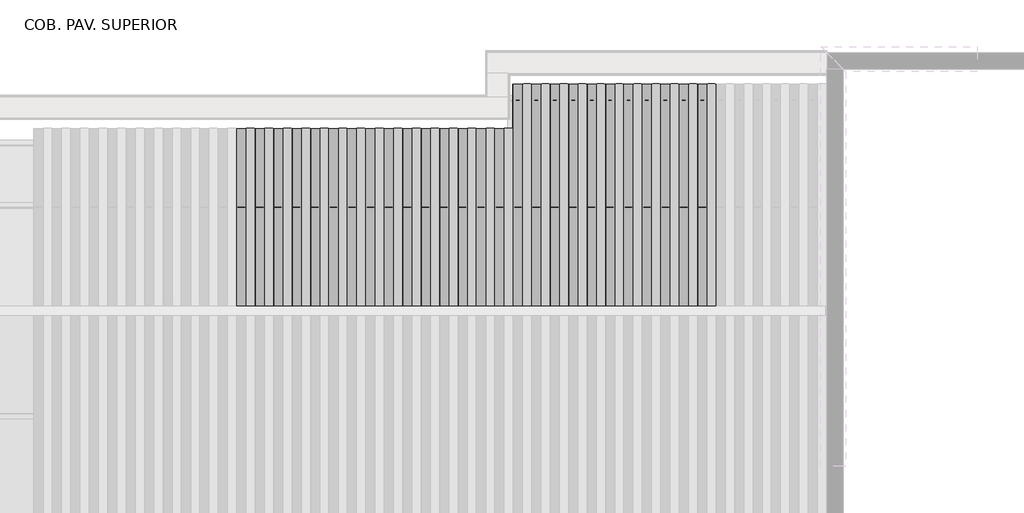
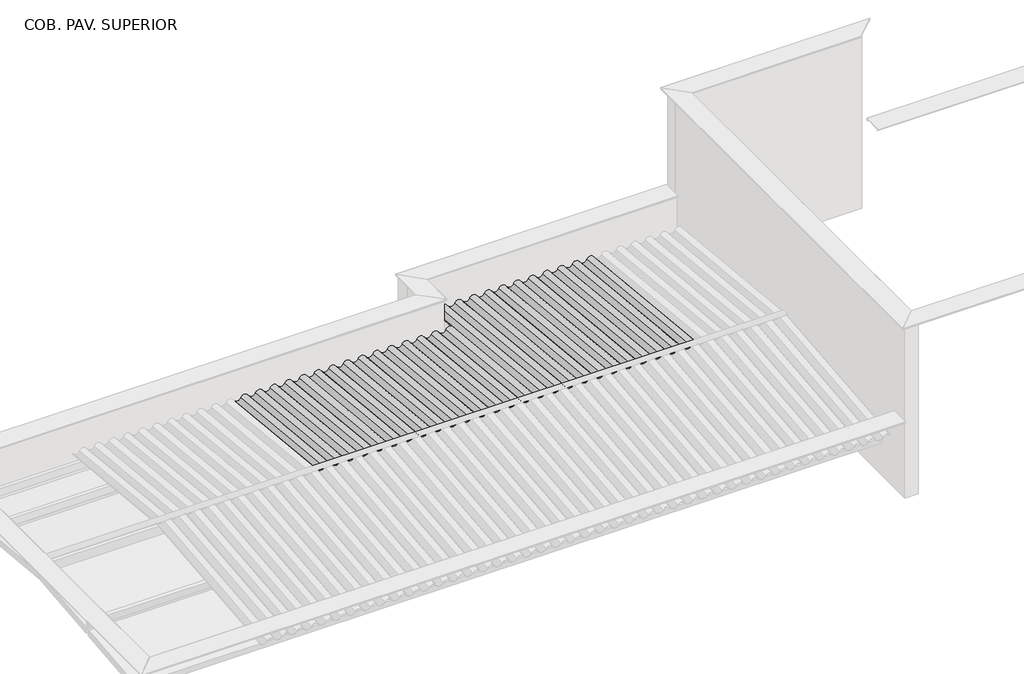
# One storey, part 4 of 7: 35 beams, 8 columns.
"""IFC4 building model written with IfcOpenShell, lengths in millimetres."""

import ifcopenshell
import ifcopenshell.guid

model = None  # the IFC model being written
_history = None  # IfcOwnerHistory: only IFC2X3 demands one
_inside = {}  # id of a spatial element -> (the spatial element, [elements in it])
_under = {}  # id of a project, library or spatial element -> (it, [spatial elements below it])
_declared = {}  # id of a project -> (the project, [libraries it declares])
_typed = {}  # id of a type object -> (the type object, [elements of that type])
_made_of = {}  # id of a material, layer set ... -> (it, [elements and type objects made of it])


def new_model(schema):
    """Start an empty IFC model of exactly this schema.

    Asked for "IFC4X3", IfcOpenShell would pick the latest addendum, in which some entities
    have other attributes; the version numbers below select the first issue.
    IFC2X3 requires an IfcOwnerHistory on every rooted entity: one is made here for all.
    """
    global model, _history
    if schema == "IFC4X3":
        model = ifcopenshell.file(schema_version=(4, 3, 0, 0))
    else:
        model = ifcopenshell.file(schema=schema)
    _inside.clear()
    _under.clear()
    _declared.clear()
    _typed.clear()
    _made_of.clear()
    _history = None
    if model.schema == "IFC2X3":
        org = make("IfcOrganization", Name="unknown")
        user = make(
            "IfcPersonAndOrganization",
            ThePerson=make("IfcPerson", FamilyName="unknown"),
            TheOrganization=org,
        )
        app = make(
            "IfcApplication",
            ApplicationDeveloper=org,
            Version="unknown",
            ApplicationFullName="unknown",
            ApplicationIdentifier="unknown",
        )
        _history = make(
            "IfcOwnerHistory",
            OwningUser=user,
            OwningApplication=app,
            ChangeAction="ADDED",
            CreationDate=0,
        )
    return model


def make(cls, **values):
    """One entity of the class cls with the attributes given. An attribute that is None is left unset."""
    return model.create_entity(
        cls, **{name: value for name, value in values.items() if value is not None}
    )


def rooted(cls, **values):
    """An entity with a GlobalId (a new one), such as an element, a storey or a relation."""
    return make(cls, GlobalId=ifcopenshell.guid.new(), OwnerHistory=_history, **values)


def si_unit(unit_type, name, prefix=None):
    """IfcSIUnit, for example si_unit("LENGTHUNIT", "METRE", prefix="MILLI")."""
    return make("IfcSIUnit", UnitType=unit_type, Prefix=prefix, Name=name)


def assignment(units):
    """IfcUnitAssignment: the units of a project."""
    return None if units is None else make("IfcUnitAssignment", Units=units)


def point(xyz):
    """IfcCartesianPoint."""
    return None if xyz is None else make("IfcCartesianPoint", Coordinates=xyz)


def direction(xyz):
    """IfcDirection."""
    return None if xyz is None else make("IfcDirection", DirectionRatios=xyz)


def frame(location, z_axis=None, x_axis=None):
    """IfcAxis2Placement3D, a coordinate frame: its origin and axes. An axis left out is left unset."""
    return make(
        "IfcAxis2Placement3D",
        Location=point(location),
        Axis=direction(z_axis),
        RefDirection=direction(x_axis),
    )


def frame_2d(location, x_axis=None):
    """IfcAxis2Placement2D, a coordinate frame in the plane: its origin and x axis."""
    return make(
        "IfcAxis2Placement2D", Location=point(location), RefDirection=direction(x_axis)
    )


def origin():
    """The frame at (0, 0, 0) with its axes left unset."""
    return frame((0.0, 0.0, 0.0))


def place(relative_to, where):
    """IfcLocalPlacement: puts the frame where relative to a parent placement (None: the world)."""
    return make(
        "IfcLocalPlacement", PlacementRelTo=relative_to, RelativePlacement=where
    )


def context(
    kind, dimensions, precision=None, world=None, true_north=None, identifier=None
):
    """IfcGeometricRepresentationContext, for example the 3D "Model" context."""
    return make(
        "IfcGeometricRepresentationContext",
        ContextIdentifier=identifier,
        ContextType=kind,
        CoordinateSpaceDimension=dimensions,
        Precision=precision,
        WorldCoordinateSystem=world,
        TrueNorth=true_north,
    )


def project(units=None, contexts=None):
    """IfcProject with its units and contexts."""
    return rooted(
        "IfcProject",
        Name="project",
        RepresentationContexts=contexts,
        UnitsInContext=assignment(units),
    )


def spatial(cls, under=None, at=None, **own):
    """A site, building, storey or space (cls), placed at a placement, below another one or the project."""
    s = rooted(cls, ObjectPlacement=at, **own)
    if under is not None:
        _under.setdefault(under.id(), (under, []))[1].append(s)
    return s


def polyline(points):
    """IfcPolyline through the points."""
    return make("IfcPolyline", Points=[point(p) for p in points])


def circle_curve(where, radius):
    """IfcCircle in the frame where."""
    return make("IfcCircle", Position=where, Radius=radius)


def trimmed(basis, trim1, trim2, sense, master):
    """IfcTrimmedCurve: the piece of a basis curve between two trims."""
    return make(
        "IfcTrimmedCurve",
        BasisCurve=basis,
        Trim1=trim1,
        Trim2=trim2,
        SenseAgreement=sense,
        MasterRepresentation=master,
    )


def segment(curve, same_sense, transition):
    """IfcCompositeCurveSegment."""
    return make(
        "IfcCompositeCurveSegment",
        Transition=transition,
        SameSense=same_sense,
        ParentCurve=curve,
    )


def composite_curve(segments, self_intersect=None):
    """IfcCompositeCurve: segments joined end to end."""
    return make("IfcCompositeCurve", Segments=segments, SelfIntersect=self_intersect)


def outline(outer, holes=None, kind="AREA"):
    """IfcArbitraryClosedProfileDef: a profile drawn as a closed curve; with holes, ...WithVoids."""
    if holes is None:
        return make("IfcArbitraryClosedProfileDef", ProfileType=kind, OuterCurve=outer)
    return make(
        "IfcArbitraryProfileDefWithVoids",
        ProfileType=kind,
        OuterCurve=outer,
        InnerCurves=holes,
    )


def extrude(swept, where, along, depth):
    """IfcExtrudedAreaSolid: the profile swept, set in the frame where, extruded along a direction by depth."""
    return make(
        "IfcExtrudedAreaSolid",
        SweptArea=swept,
        Position=where,
        ExtrudedDirection=direction(along),
        Depth=depth,
    )


def shape(context_of_items, identifier, shape_type, items):
    """IfcShapeRepresentation: the items that make up one representation, for example the "Body"."""
    return make(
        "IfcShapeRepresentation",
        ContextOfItems=context_of_items,
        RepresentationIdentifier=identifier,
        RepresentationType=shape_type,
        Items=items,
    )


def source(mapping_origin, context_of_items, identifier, shape_type, items):
    """IfcRepresentationMap: a shape defined once, which mapped items show again and again."""
    return make(
        "IfcRepresentationMap",
        MappingOrigin=mapping_origin,
        MappedRepresentation=shape(context_of_items, identifier, shape_type, items),
    )


def transform(
    local_origin,
    x_axis=None,
    y_axis=None,
    z_axis=None,
    scale=None,
    scale2=None,
    scale3=None,
    uniform=True,
):
    """IfcCartesianTransformationOperator3D, or its non-uniform kind. x_axis, y_axis, z_axis: its Axis1, 2, 3."""
    if uniform:
        return make(
            "IfcCartesianTransformationOperator3D",
            Axis1=direction(x_axis),
            Axis2=direction(y_axis),
            LocalOrigin=point(local_origin),
            Scale=scale,
            Axis3=direction(z_axis),
        )
    return make(
        "IfcCartesianTransformationOperator3DnonUniform",
        Axis1=direction(x_axis),
        Axis2=direction(y_axis),
        LocalOrigin=point(local_origin),
        Scale=scale,
        Axis3=direction(z_axis),
        Scale2=scale2,
        Scale3=scale3,
    )


def mapped(mapping_source, mapping_target):
    """IfcMappedItem: shows the shape of a source again, moved by a transform."""
    return make(
        "IfcMappedItem", MappingSource=mapping_source, MappingTarget=mapping_target
    )


def made_of(thing, what):
    """Note that an element or type object is made of a material, layer set ...; save() writes the relation."""
    if what is not None:
        _made_of.setdefault(what.id(), (what, []))[1].append(thing)
    return thing


def element(
    cls,
    number,
    at=None,
    inside=None,
    cuts=None,
    type_object=None,
    material=None,
    context=None,
    identifier="Body",
    shape_type=None,
    held_by="IfcProductDefinitionShape",
    body=None,
    shapes=None,
    **own,
):
    """One element of the class cls, such as IfcWall. Its Tag is "e" and its number.

    at: its placement. inside: the storey or other place that contains it. cuts: it is an
    opening in that element (IfcRelVoidsElement). A single representation is given by context,
    identifier, shape_type and body (its items); several are given by shapes. held_by: the class
    of the entity that holds the representations. save() writes the other relations.
    """
    e = rooted(cls, Tag="e%d" % number, ObjectPlacement=at, **own)
    if body is not None:
        shapes = [shape(context, identifier, shape_type, body)]
    if shapes is not None:
        e.Representation = make(held_by, Representations=shapes)
    if inside is not None:
        _inside.setdefault(inside.id(), (inside, []))[1].append(e)
    if cuts is not None:
        rooted(
            "IfcRelVoidsElement", RelatingBuildingElement=cuts, RelatedOpeningElement=e
        )
    if type_object is not None:
        _typed.setdefault(type_object.id(), (type_object, []))[1].append(e)
    return made_of(e, material)


def aggregate(whole, parts):
    """IfcRelAggregates: a whole, such as a stair, and the parts it consists of."""
    return rooted("IfcRelAggregates", RelatingObject=whole, RelatedObjects=parts)


def save(model, path):
    """Write the relations noted so far, then the file.

    IfcRelAggregates (storeys below a building ...), IfcRelContainedInSpatialStructure (elements
    in a storey), IfcRelDefinesByType, IfcRelAssociatesMaterial and IfcRelDeclares: one each for
    every whole, place, type object, material and project.
    """
    for whole, parts in _under.values():
        aggregate(whole, parts)
    for where, things in _inside.values():
        rooted(
            "IfcRelContainedInSpatialStructure",
            RelatedElements=things,
            RelatingStructure=where,
        )
    for kind, things in _typed.values():
        rooted("IfcRelDefinesByType", RelatedObjects=things, RelatingType=kind)
    for what, things in _made_of.values():
        rooted("IfcRelAssociatesMaterial", RelatedObjects=things, RelatingMaterial=what)
    for by, libraries in _declared.values():
        rooted("IfcRelDeclares", RelatingContext=by, RelatedDefinitions=libraries)
    model.write(path)


def column_d505325c(model_context):
    return source(origin(), model_context, "Body", "SweptSolid", [
        extrude(outline(polyline([(30.0, 80.0), (30.0, -80.0), (-30.0, -80.0), (-30.0, 80.0), (30.0, 80.0)])), frame((0.0, 0.0, 6710.0), z_axis=(0.0, 0.0, 1.0), x_axis=(1.0, 0.0, 0.0)), (0.0, 0.0, 1.0), 750.0),
    ])


def column_df674f92(model_context):
    return source(origin(), model_context, "Body", "SweptSolid", [
        extrude(outline(polyline([(30.0, 80.0), (30.0, -80.0), (-30.0, -80.0), (-30.0, 80.0), (30.0, 80.0)])), frame((0.0, 0.0, 6710.0), z_axis=(0.0, 0.0, 1.0), x_axis=(1.0, 0.0, 0.0)), (0.0, 0.0, 1.0), 575.0),
    ])


def column_4db371bd(model_context):
    return source(origin(), model_context, "Body", "SweptSolid", [
        extrude(outline(polyline([(30.0, 80.0), (30.0, -80.0), (-30.0, -80.0), (-30.0, 80.0), (30.0, 80.0)])), frame((0.0, 0.0, 6710.0), z_axis=(0.0, 0.0, 1.0), x_axis=(1.0, 0.0, 0.0)), (0.0, 0.0, 1.0), 660.0),
    ])


model = new_model("IFC4")

# Units and contexts
model_context = context("Model", 3, world=origin())
ifc_project = project(units=[si_unit("LENGTHUNIT", "METRE", prefix="MILLI")], contexts=[model_context])

# Site, building, storey
site = spatial("IfcSite", under=ifc_project)
building = spatial("IfcBuilding", under=site)
storey = spatial("IfcBuildingStorey", under=building, Name="COB. PAV. SUPERIOR", Elevation=6650.0)

# Beams
placement = place(None, origin())
element("IfcBeam", 1, ObjectType="Madeira de lei : Berço 6x12cm", at=placement, inside=storey, context=model_context, shape_type="SweptSolid", body=[
    extrude(outline(polyline([(-4679.281307, -7711.5607799), (-4679.281307, -7831.5607799), (-6679.281307, -7831.5607799), (-6679.281307, -7711.5607799), (-4679.281307, -7711.5607799)])), frame((0.0, 0.0, 6650.0), z_axis=(0.0, 0.0, 1.0), x_axis=(1.0, 0.0, 0.0)), (0.0, 0.0, 1.0), 60.0),
])
element("IfcBeam", 2, ObjectType="Madeira de lei : Berço 6x12cm", at=placement, inside=storey, context=model_context, shape_type="SweptSolid", body=[
    extrude(outline(polyline([(-2679.281307, -7711.5607799), (-2679.281307, -7831.5607799), (-4679.281307, -7831.5607799), (-4679.281307, -7711.5607799), (-2679.281307, -7711.5607799)])), frame((0.0, 0.0, 6650.0), z_axis=(0.0, 0.0, 1.0), x_axis=(1.0, 0.0, 0.0)), (0.0, 0.0, 1.0), 60.0),
])
element("IfcBeam", 3, ObjectType="Madeira de lei : Berço 6x12cm", at=placement, inside=storey, context=model_context, shape_type="SweptSolid", body=[
    extrude(outline(polyline([(-679.281307, -7711.5607799), (-679.281307, -7831.5607799), (-2679.281307, -7831.5607799), (-2679.281307, -7711.5607799), (-679.281307, -7711.5607799)])), frame((0.0, 0.0, 6650.0), z_axis=(0.0, 0.0, 1.0), x_axis=(1.0, 0.0, 0.0)), (0.0, 0.0, 1.0), 60.0),
])
element("IfcBeam", 4, ObjectType="Madeira de lei : Berço 6x12cm", at=placement, inside=storey, context=model_context, shape_type="SweptSolid", body=[
    extrude(outline(polyline([(-244.281307, -7711.5607799), (-244.281307, -7831.5607799), (-679.281307, -7831.5607799), (-679.281307, -7711.5607799), (-244.281307, -7711.5607799)])), frame((0.0, 0.0, 6650.0), z_axis=(0.0, 0.0, 1.0), x_axis=(1.0, 0.0, 0.0)), (0.0, 0.0, 1.0), 60.0),
])
element("IfcBeam", 5, ObjectType="Madeira de lei : Berço 6x12cm", at=placement, inside=storey, context=model_context, shape_type="SweptSolid", body=[
    extrude(outline(polyline([(-6779.2813076, -5488.3211004), (-6779.2813076, -5608.3211004), (-8589.281307, -5608.3211004), (-8589.281307, -5488.3211004), (-6779.2813076, -5488.3211004)])), frame((0.0, 0.0, 6650.0), z_axis=(0.0, 0.0, 1.0), x_axis=(1.0, 0.0, 0.0)), (0.0, 0.0, 1.0), 60.0),
])
element("IfcBeam", 6, ObjectType="Madeira de lei : Berço 6x12cm", at=placement, inside=storey, context=model_context, shape_type="SweptSolid", body=[
    extrude(outline(polyline([(-4779.281307, -5488.3211004), (-4779.281307, -5608.3211004), (-6779.2813063, -5608.3211004), (-6779.2813063, -5488.3211004), (-4779.281307, -5488.3211004)])), frame((0.0, 0.0, 6650.0), z_axis=(0.0, 0.0, 1.0), x_axis=(1.0, 0.0, 0.0)), (0.0, 0.0, 1.0), 60.0),
])
element("IfcBeam", 7, ObjectType="Madeira de lei : Berço 6x12cm", at=placement, inside=storey, context=model_context, shape_type="SweptSolid", body=[
    extrude(outline(polyline([(-6840.281307, -6319.8711004), (-6840.281307, -6439.8711004), (-8589.281307, -6439.8711004), (-8589.281307, -6319.8711004), (-6840.281307, -6319.8711004)])), frame((0.0, 0.0, 6650.0), z_axis=(0.0, 0.0, 1.0), x_axis=(1.0, 0.0, 0.0)), (0.0, 0.0, 1.0), 60.0),
])
element("IfcBeam", 8, ObjectType="Madeira de lei : Berço 6x12cm", at=placement, inside=storey, context=model_context, shape_type="SweptSolid", body=[
    extrude(outline(polyline([(-4679.2813076, -6319.8711004), (-4679.2813076, -6439.8711004), (-6440.281307, -6439.8711004), (-6440.281307, -6319.8711004), (-4679.2813076, -6319.8711004)])), frame((0.0, 0.0, 6650.0), z_axis=(0.0, 0.0, 1.0), x_axis=(1.0, 0.0, 0.0)), (0.0, 0.0, 1.0), 60.0),
])
element("IfcBeam", 9, ObjectType="Madeira de lei : Berço 6x12cm", at=placement, inside=storey, context=model_context, shape_type="SweptSolid", body=[
    extrude(outline(polyline([(-2679.2813076, -6319.8711004), (-2679.2813076, -6439.8711004), (-4679.2813064, -6439.8711004), (-4679.2813064, -6319.8711004), (-2679.2813076, -6319.8711004)])), frame((0.0, 0.0, 6650.0), z_axis=(0.0, 0.0, 1.0), x_axis=(1.0, 0.0, 0.0)), (0.0, 0.0, 1.0), 60.0),
])
element("IfcBeam", 10, ObjectType="Telha Ondulada : Fibrocimento", at=placement, inside=storey, context=model_context, shape_type="SweptSolid", body=[
    extrude(outline(composite_curve([segment(trimmed(circle_curve(frame_2d((-58.7002978, -53.2060539)), 66.7939461), [point((-29.3501489, 6.7939461))], [point((-29.3501489, -113.2060539))], False, "CARTESIAN"), True, "CONTINUOUS"), segment(polyline([(-29.3501489, -113.2060539), (-31.5472154, -108.7146289)]), True, "CONTINUOUS"), segment(trimmed(circle_curve(frame_2d((-58.7002978, -53.2060539)), 61.7939461), [point((-31.5472154, -108.7146289))], [point((-31.5472154, 2.3025211))], True, "CARTESIAN"), True, "CONTINUOUS"), segment(trimmed(circle_curve(frame_2d((0.0, 66.7939461)), 71.7939461), [point((-31.5472154, 2.3025211))], [point((-31.5472154, 131.2853711))], False, "CARTESIAN"), True, "CONTINUOUS"), segment(polyline([(-31.5472154, 131.2853711), (-29.3501489, 126.7939461)]), True, "CONTINUOUS"), segment(trimmed(circle_curve(frame_2d((0.0, 66.7939461)), 66.7939461), [point((-29.3501489, 126.7939461))], [point((-29.3501489, 6.7939461))], True, "CARTESIAN"), True, "CONTINUOUS")], self_intersect=False)), frame((-7939.8843743, -5348.1805671, 7453.4315886), z_axis=(0.0, -0.9950371902099893, 0.09950371902099772), x_axis=(0.0, 0.09950371902099772, 0.9950371902099893)), (0.0, 0.0, 1.0), 2425.2918406),
])
element("IfcBeam", 11, ObjectType="Telha Ondulada : Fibrocimento", at=placement, inside=storey, context=model_context, shape_type="SweptSolid", body=[
    extrude(outline(composite_curve([segment(trimmed(circle_curve(frame_2d((-58.7002978, -53.2060539)), 66.7939461), [point((-29.3501489, 6.7939461))], [point((-29.3501489, -113.2060539))], False, "CARTESIAN"), True, "CONTINUOUS"), segment(polyline([(-29.3501489, -113.2060539), (-31.5472154, -108.7146289)]), True, "CONTINUOUS"), segment(trimmed(circle_curve(frame_2d((-58.7002978, -53.2060539)), 61.7939461), [point((-31.5472154, -108.7146289))], [point((-31.5472154, 2.3025211))], True, "CARTESIAN"), True, "CONTINUOUS"), segment(trimmed(circle_curve(frame_2d((0.0, 66.7939461)), 71.7939461), [point((-31.5472154, 2.3025211))], [point((-31.5472154, 131.2853711))], False, "CARTESIAN"), True, "CONTINUOUS"), segment(polyline([(-31.5472154, 131.2853711), (-29.3501489, 126.7939461)]), True, "CONTINUOUS"), segment(trimmed(circle_curve(frame_2d((0.0, 66.7939461)), 66.7939461), [point((-29.3501489, 126.7939461))], [point((-29.3501489, 6.7939461))], True, "CARTESIAN"), True, "CONTINUOUS")], self_intersect=False)), frame((-7695.3843743, -5348.1805671, 7453.4315886), z_axis=(0.0, -0.9950371902099893, 0.09950371902099772), x_axis=(0.0, 0.09950371902099772, 0.9950371902099893)), (0.0, 0.0, 1.0), 2425.2918406),
])
element("IfcBeam", 12, ObjectType="Telha Ondulada : Fibrocimento", at=placement, inside=storey, context=model_context, shape_type="SweptSolid", body=[
    extrude(outline(composite_curve([segment(trimmed(circle_curve(frame_2d((-58.7002978, -53.2060539)), 66.7939461), [point((-29.3501489, 6.7939461))], [point((-29.3501489, -113.2060539))], False, "CARTESIAN"), True, "CONTINUOUS"), segment(polyline([(-29.3501489, -113.2060539), (-31.5472154, -108.7146289)]), True, "CONTINUOUS"), segment(trimmed(circle_curve(frame_2d((-58.7002978, -53.2060539)), 61.7939461), [point((-31.5472154, -108.7146289))], [point((-31.5472154, 2.3025211))], True, "CARTESIAN"), True, "CONTINUOUS"), segment(trimmed(circle_curve(frame_2d((0.0, 66.7939461)), 71.7939461), [point((-31.5472154, 2.3025211))], [point((-31.5472154, 131.2853711))], False, "CARTESIAN"), True, "CONTINUOUS"), segment(polyline([(-31.5472154, 131.2853711), (-29.3501489, 126.7939461)]), True, "CONTINUOUS"), segment(trimmed(circle_curve(frame_2d((0.0, 66.7939461)), 66.7939461), [point((-29.3501489, 126.7939461))], [point((-29.3501489, 6.7939461))], True, "CARTESIAN"), True, "CONTINUOUS")], self_intersect=False)), frame((-7450.8843743, -5348.1805671, 7453.4315886), z_axis=(0.0, -0.9950371902099893, 0.09950371902099768), x_axis=(0.0, 0.09950371902099768, 0.9950371902099893)), (0.0, 0.0, 1.0), 2425.2918406),
])
element("IfcBeam", 13, ObjectType="Telha Ondulada : Fibrocimento", at=placement, inside=storey, context=model_context, shape_type="SweptSolid", body=[
    extrude(outline(composite_curve([segment(trimmed(circle_curve(frame_2d((-58.7002978, -53.2060539)), 66.7939461), [point((-29.3501489, 6.7939461))], [point((-29.3501489, -113.2060539))], False, "CARTESIAN"), True, "CONTINUOUS"), segment(polyline([(-29.3501489, -113.2060539), (-31.5472154, -108.7146289)]), True, "CONTINUOUS"), segment(trimmed(circle_curve(frame_2d((-58.7002978, -53.2060539)), 61.7939461), [point((-31.5472154, -108.7146289))], [point((-31.5472154, 2.3025211))], True, "CARTESIAN"), True, "CONTINUOUS"), segment(trimmed(circle_curve(frame_2d((0.0, 66.7939461)), 71.7939461), [point((-31.5472154, 2.3025211))], [point((-31.5472154, 131.2853711))], False, "CARTESIAN"), True, "CONTINUOUS"), segment(polyline([(-31.5472154, 131.2853711), (-29.3501489, 126.7939461)]), True, "CONTINUOUS"), segment(trimmed(circle_curve(frame_2d((0.0, 66.7939461)), 66.7939461), [point((-29.3501489, 126.7939461))], [point((-29.3501489, 6.7939461))], True, "CARTESIAN"), True, "CONTINUOUS")], self_intersect=False)), frame((-7206.3843743, -5348.1805671, 7453.4315886), z_axis=(0.0, -0.9950371902099893, 0.09950371902099768), x_axis=(0.0, 0.09950371902099768, 0.9950371902099893)), (0.0, 0.0, 1.0), 2425.2918406),
])
element("IfcBeam", 14, ObjectType="Telha Ondulada : Fibrocimento", at=placement, inside=storey, context=model_context, shape_type="SweptSolid", body=[
    extrude(outline(composite_curve([segment(trimmed(circle_curve(frame_2d((-58.7002978, -53.2060539)), 66.7939461), [point((-29.3501489, 6.7939461))], [point((-29.3501489, -113.2060539))], False, "CARTESIAN"), True, "CONTINUOUS"), segment(polyline([(-29.3501489, -113.2060539), (-31.5472154, -108.7146289)]), True, "CONTINUOUS"), segment(trimmed(circle_curve(frame_2d((-58.7002978, -53.2060539)), 61.7939461), [point((-31.5472154, -108.7146289))], [point((-31.5472154, 2.3025211))], True, "CARTESIAN"), True, "CONTINUOUS"), segment(trimmed(circle_curve(frame_2d((0.0, 66.7939461)), 71.7939461), [point((-31.5472154, 2.3025211))], [point((-31.5472154, 131.2853711))], False, "CARTESIAN"), True, "CONTINUOUS"), segment(polyline([(-31.5472154, 131.2853711), (-29.3501489, 126.7939461)]), True, "CONTINUOUS"), segment(trimmed(circle_curve(frame_2d((0.0, 66.7939461)), 66.7939461), [point((-29.3501489, 126.7939461))], [point((-29.3501489, 6.7939461))], True, "CARTESIAN"), True, "CONTINUOUS")], self_intersect=False)), frame((-6961.8843743, -5348.1805671, 7453.4315886), z_axis=(0.0, -0.9950371902099893, 0.09950371902099768), x_axis=(0.0, 0.09950371902099768, 0.9950371902099893)), (0.0, 0.0, 1.0), 2425.2918406),
])
element("IfcBeam", 15, ObjectType="Telha Ondulada : Fibrocimento", at=placement, inside=storey, context=model_context, shape_type="SweptSolid", body=[
    extrude(outline(composite_curve([segment(trimmed(circle_curve(frame_2d((-58.7002978, -53.2060539)), 66.7939461), [point((-29.3501489, 6.7939461))], [point((-29.3501489, -113.2060539))], False, "CARTESIAN"), True, "CONTINUOUS"), segment(polyline([(-29.3501489, -113.2060539), (-31.5472154, -108.7146289)]), True, "CONTINUOUS"), segment(trimmed(circle_curve(frame_2d((-58.7002978, -53.2060539)), 61.7939461), [point((-31.5472154, -108.7146289))], [point((-31.5472154, 2.3025211))], True, "CARTESIAN"), True, "CONTINUOUS"), segment(trimmed(circle_curve(frame_2d((0.0, 66.7939461)), 71.7939461), [point((-31.5472154, 2.3025211))], [point((-31.5472154, 131.2853711))], False, "CARTESIAN"), True, "CONTINUOUS"), segment(polyline([(-31.5472154, 131.2853711), (-29.3501489, 126.7939461)]), True, "CONTINUOUS"), segment(trimmed(circle_curve(frame_2d((0.0, 66.7939461)), 66.7939461), [point((-29.3501489, 126.7939461))], [point((-29.3501489, 6.7939461))], True, "CARTESIAN"), True, "CONTINUOUS")], self_intersect=False)), frame((-6717.3843743, -5348.1805671, 7453.4315886), z_axis=(0.0, -0.9950371902099893, 0.09950371902099768), x_axis=(0.0, 0.09950371902099768, 0.9950371902099893)), (0.0, 0.0, 1.0), 2425.2918406),
])
element("IfcBeam", 16, ObjectType="Telha Ondulada : Fibrocimento", at=placement, inside=storey, context=model_context, shape_type="SweptSolid", body=[
    extrude(outline(composite_curve([segment(trimmed(circle_curve(frame_2d((-58.7002978, -53.2060539)), 66.7939461), [point((-29.3501489, 6.7939461))], [point((-29.3501489, -113.2060539))], False, "CARTESIAN"), True, "CONTINUOUS"), segment(polyline([(-29.3501489, -113.2060539), (-31.5472154, -108.7146289)]), True, "CONTINUOUS"), segment(trimmed(circle_curve(frame_2d((-58.7002978, -53.2060539)), 61.7939461), [point((-31.5472154, -108.7146289))], [point((-31.5472154, 2.3025211))], True, "CARTESIAN"), True, "CONTINUOUS"), segment(trimmed(circle_curve(frame_2d((0.0, 66.7939461)), 71.7939461), [point((-31.5472154, 2.3025211))], [point((-31.5472154, 131.2853711))], False, "CARTESIAN"), True, "CONTINUOUS"), segment(polyline([(-31.5472154, 131.2853711), (-29.3501489, 126.7939461)]), True, "CONTINUOUS"), segment(trimmed(circle_curve(frame_2d((0.0, 66.7939461)), 66.7939461), [point((-29.3501489, 126.7939461))], [point((-29.3501489, 6.7939461))], True, "CARTESIAN"), True, "CONTINUOUS")], self_intersect=False)), frame((-6472.8843743, -5348.1805671, 7453.4315886), z_axis=(0.0, -0.9950371902099893, 0.09950371902099772), x_axis=(0.0, 0.09950371902099772, 0.9950371902099893)), (0.0, 0.0, 1.0), 2425.2918406),
])
element("IfcBeam", 17, ObjectType="Telha Ondulada : Fibrocimento", at=placement, inside=storey, context=model_context, shape_type="SweptSolid", body=[
    extrude(outline(composite_curve([segment(trimmed(circle_curve(frame_2d((-58.7002978, -53.2060539)), 66.7939461), [point((-29.3501489, 6.7939461))], [point((-29.3501489, -113.2060539))], False, "CARTESIAN"), True, "CONTINUOUS"), segment(polyline([(-29.3501489, -113.2060539), (-31.5472154, -108.7146289)]), True, "CONTINUOUS"), segment(trimmed(circle_curve(frame_2d((-58.7002978, -53.2060539)), 61.7939461), [point((-31.5472154, -108.7146289))], [point((-31.5472154, 2.3025211))], True, "CARTESIAN"), True, "CONTINUOUS"), segment(trimmed(circle_curve(frame_2d((0.0, 66.7939461)), 71.7939461), [point((-31.5472154, 2.3025211))], [point((-31.5472154, 131.2853711))], False, "CARTESIAN"), True, "CONTINUOUS"), segment(polyline([(-31.5472154, 131.2853711), (-29.3501489, 126.7939461)]), True, "CONTINUOUS"), segment(trimmed(circle_curve(frame_2d((0.0, 66.7939461)), 66.7939461), [point((-29.3501489, 126.7939461))], [point((-29.3501489, 6.7939461))], True, "CARTESIAN"), True, "CONTINUOUS")], self_intersect=False)), frame((-6228.3843743, -5348.1805671, 7453.4315886), z_axis=(0.0, -0.9950371902099893, 0.09950371902099768), x_axis=(0.0, 0.09950371902099768, 0.9950371902099893)), (0.0, 0.0, 1.0), 2425.2918406),
])
element("IfcBeam", 18, ObjectType="Telha Ondulada : Fibrocimento", at=placement, inside=storey, context=model_context, shape_type="SweptSolid", body=[
    extrude(outline(composite_curve([segment(trimmed(circle_curve(frame_2d((-58.7002978, -53.2060539)), 66.7939461), [point((-29.3501489, 6.7939461))], [point((-29.3501489, -113.2060539))], False, "CARTESIAN"), True, "CONTINUOUS"), segment(polyline([(-29.3501489, -113.2060539), (-31.5472154, -108.7146289)]), True, "CONTINUOUS"), segment(trimmed(circle_curve(frame_2d((-58.7002978, -53.2060539)), 61.7939461), [point((-31.5472154, -108.7146289))], [point((-31.5472154, 2.3025211))], True, "CARTESIAN"), True, "CONTINUOUS"), segment(trimmed(circle_curve(frame_2d((0.0, 66.7939461)), 71.7939461), [point((-31.5472154, 2.3025211))], [point((-31.5472154, 131.2853711))], False, "CARTESIAN"), True, "CONTINUOUS"), segment(polyline([(-31.5472154, 131.2853711), (-29.3501489, 126.7939461)]), True, "CONTINUOUS"), segment(trimmed(circle_curve(frame_2d((0.0, 66.7939461)), 66.7939461), [point((-29.3501489, 126.7939461))], [point((-29.3501489, 6.7939461))], True, "CARTESIAN"), True, "CONTINUOUS")], self_intersect=False)), frame((-5983.8843743, -5348.1805671, 7453.4315886), z_axis=(0.0, -0.9950371902099893, 0.09950371902099772), x_axis=(0.0, 0.09950371902099772, 0.9950371902099893)), (0.0, 0.0, 1.0), 2425.2918406),
])
element("IfcBeam", 19, ObjectType="Telha Ondulada : Fibrocimento", at=placement, inside=storey, context=model_context, shape_type="SweptSolid", body=[
    extrude(outline(composite_curve([segment(trimmed(circle_curve(frame_2d((-58.7002978, -53.2060539)), 66.7939461), [point((-29.3501489, 6.7939461))], [point((-29.3501489, -113.2060539))], False, "CARTESIAN"), True, "CONTINUOUS"), segment(polyline([(-29.3501489, -113.2060539), (-31.5472154, -108.7146289)]), True, "CONTINUOUS"), segment(trimmed(circle_curve(frame_2d((-58.7002978, -53.2060539)), 61.7939461), [point((-31.5472154, -108.7146289))], [point((-31.5472154, 2.3025211))], True, "CARTESIAN"), True, "CONTINUOUS"), segment(trimmed(circle_curve(frame_2d((0.0, 66.7939461)), 71.7939461), [point((-31.5472154, 2.3025211))], [point((-31.5472154, 131.2853711))], False, "CARTESIAN"), True, "CONTINUOUS"), segment(polyline([(-31.5472154, 131.2853711), (-29.3501489, 126.7939461)]), True, "CONTINUOUS"), segment(trimmed(circle_curve(frame_2d((0.0, 66.7939461)), 66.7939461), [point((-29.3501489, 126.7939461))], [point((-29.3501489, 6.7939461))], True, "CARTESIAN"), True, "CONTINUOUS")], self_intersect=False)), frame((-5739.3843743, -5348.1805671, 7453.4315886), z_axis=(0.0, -0.9950371902099893, 0.09950371902099772), x_axis=(0.0, 0.09950371902099772, 0.9950371902099893)), (0.0, 0.0, 1.0), 2425.2918406),
])
element("IfcBeam", 20, ObjectType="Telha Ondulada : Fibrocimento", at=placement, inside=storey, context=model_context, shape_type="SweptSolid", body=[
    extrude(outline(composite_curve([segment(trimmed(circle_curve(frame_2d((-58.7002978, -53.2060539)), 66.7939461), [point((-29.3501489, 6.7939461))], [point((-29.3501489, -113.2060539))], False, "CARTESIAN"), True, "CONTINUOUS"), segment(polyline([(-29.3501489, -113.2060539), (-31.5472154, -108.7146289)]), True, "CONTINUOUS"), segment(trimmed(circle_curve(frame_2d((-58.7002978, -53.2060539)), 61.7939461), [point((-31.5472154, -108.7146289))], [point((-31.5472154, 2.3025211))], True, "CARTESIAN"), True, "CONTINUOUS"), segment(trimmed(circle_curve(frame_2d((0.0, 66.7939461)), 71.7939461), [point((-31.5472154, 2.3025211))], [point((-31.5472154, 131.2853711))], False, "CARTESIAN"), True, "CONTINUOUS"), segment(polyline([(-31.5472154, 131.2853711), (-29.3501489, 126.7939461)]), True, "CONTINUOUS"), segment(trimmed(circle_curve(frame_2d((0.0, 66.7939461)), 66.7939461), [point((-29.3501489, 126.7939461))], [point((-29.3501489, 6.7939461))], True, "CARTESIAN"), True, "CONTINUOUS")], self_intersect=False)), frame((-5494.8843743, -5348.1805671, 7453.4315886), z_axis=(0.0, -0.9950371902099893, 0.09950371902099768), x_axis=(0.0, 0.09950371902099768, 0.9950371902099893)), (0.0, 0.0, 1.0), 2425.2918406),
])
element("IfcBeam", 21, ObjectType="Telha Ondulada : Fibrocimento", at=placement, inside=storey, context=model_context, shape_type="SweptSolid", body=[
    extrude(outline(composite_curve([segment(trimmed(circle_curve(frame_2d((-58.7002978, -53.2060539)), 66.7939461), [point((-29.3501489, 6.7939461))], [point((-29.3501489, -113.2060539))], False, "CARTESIAN"), True, "CONTINUOUS"), segment(polyline([(-29.3501489, -113.2060539), (-31.5472154, -108.7146289)]), True, "CONTINUOUS"), segment(trimmed(circle_curve(frame_2d((-58.7002978, -53.2060539)), 61.7939461), [point((-31.5472154, -108.7146289))], [point((-31.5472154, 2.3025211))], True, "CARTESIAN"), True, "CONTINUOUS"), segment(trimmed(circle_curve(frame_2d((0.0, 66.7939461)), 71.7939461), [point((-31.5472154, 2.3025211))], [point((-31.5472154, 131.2853711))], False, "CARTESIAN"), True, "CONTINUOUS"), segment(polyline([(-31.5472154, 131.2853711), (-29.3501489, 126.7939461)]), True, "CONTINUOUS"), segment(trimmed(circle_curve(frame_2d((0.0, 66.7939461)), 66.7939461), [point((-29.3501489, 126.7939461))], [point((-29.3501489, 6.7939461))], True, "CARTESIAN"), True, "CONTINUOUS")], self_intersect=False)), frame((-5250.3843743, -5348.1805671, 7453.4315886), z_axis=(0.0, -0.9950371902099893, 0.09950371902099772), x_axis=(0.0, 0.09950371902099772, 0.9950371902099893)), (0.0, 0.0, 1.0), 2425.2918406),
])
element("IfcBeam", 22, ObjectType="Telha Ondulada : Fibrocimento", at=placement, inside=storey, context=model_context, shape_type="SweptSolid", body=[
    extrude(outline(composite_curve([segment(trimmed(circle_curve(frame_2d((-58.7002978, -53.2060539)), 66.7939461), [point((-29.3501489, 6.7939461))], [point((-29.3501489, -113.2060539))], False, "CARTESIAN"), True, "CONTINUOUS"), segment(polyline([(-29.3501489, -113.2060539), (-31.5472154, -108.7146289)]), True, "CONTINUOUS"), segment(trimmed(circle_curve(frame_2d((-58.7002978, -53.2060539)), 61.7939461), [point((-31.5472154, -108.7146289))], [point((-31.5472154, 2.3025211))], True, "CARTESIAN"), True, "CONTINUOUS"), segment(trimmed(circle_curve(frame_2d((0.0, 66.7939461)), 71.7939461), [point((-31.5472154, 2.3025211))], [point((-31.5472154, 131.2853711))], False, "CARTESIAN"), True, "CONTINUOUS"), segment(polyline([(-31.5472154, 131.2853711), (-29.3501489, 126.7939461)]), True, "CONTINUOUS"), segment(trimmed(circle_curve(frame_2d((0.0, 66.7939461)), 66.7939461), [point((-29.3501489, 126.7939461))], [point((-29.3501489, 6.7939461))], True, "CARTESIAN"), True, "CONTINUOUS")], self_intersect=False)), frame((-5005.8843743, -5348.1805671, 7453.4315886), z_axis=(0.0, -0.9950371902099893, 0.09950371902099772), x_axis=(0.0, 0.09950371902099772, 0.9950371902099893)), (0.0, 0.0, 1.0), 2425.2918406),
])
element("IfcBeam", 23, ObjectType="Telha Ondulada : Fibrocimento", at=placement, inside=storey, context=model_context, shape_type="SweptSolid", body=[
    extrude(outline(composite_curve([segment(trimmed(circle_curve(frame_2d((-58.7002978, -53.2060539)), 66.7939461), [point((-29.3501489, 6.7939461))], [point((-29.3501489, -113.2060539))], False, "CARTESIAN"), True, "CONTINUOUS"), segment(polyline([(-29.3501489, -113.2060539), (-31.5472154, -108.7146289)]), True, "CONTINUOUS"), segment(trimmed(circle_curve(frame_2d((-58.7002978, -53.2060539)), 61.7939461), [point((-31.5472154, -108.7146289))], [point((-31.5472154, 2.3025211))], True, "CARTESIAN"), True, "CONTINUOUS"), segment(trimmed(circle_curve(frame_2d((0.0, 66.7939461)), 71.7939461), [point((-31.5472154, 2.3025211))], [point((-31.5472154, 131.2853711))], False, "CARTESIAN"), True, "CONTINUOUS"), segment(polyline([(-31.5472154, 131.2853711), (-29.3501489, 126.7939461)]), True, "CONTINUOUS"), segment(trimmed(circle_curve(frame_2d((0.0, 66.7939461)), 66.7939461), [point((-29.3501489, 126.7939461))], [point((-29.3501489, 6.7939461))], True, "CARTESIAN"), True, "CONTINUOUS")], self_intersect=False)), frame((-4761.3843743, -5348.1805671, 7453.4315886), z_axis=(0.0, -0.9950371902099893, 0.09950371902099768), x_axis=(0.0, 0.09950371902099768, 0.9950371902099893)), (0.0, 0.0, 1.0), 2425.2918406),
])
element("IfcBeam", 24, ObjectType="Telha Ondulada : Fibrocimento", at=placement, inside=storey, context=model_context, shape_type="SweptSolid", body=[
    extrude(outline(composite_curve([segment(trimmed(circle_curve(frame_2d((-58.7002978, -53.2060539)), 66.7939461), [point((-29.3501489, 6.7939461))], [point((-29.3501489, -113.2060539))], False, "CARTESIAN"), True, "CONTINUOUS"), segment(polyline([(-29.3501489, -113.2060539), (-31.5472154, -108.7146289)]), True, "CONTINUOUS"), segment(trimmed(circle_curve(frame_2d((-58.7002978, -53.2060539)), 61.7939461), [point((-31.5472154, -108.7146289))], [point((-31.5472154, 2.3025211))], True, "CARTESIAN"), True, "CONTINUOUS"), segment(trimmed(circle_curve(frame_2d((0.0, 66.7939461)), 71.7939461), [point((-31.5472154, 2.3025211))], [point((-31.5472154, 131.2853711))], False, "CARTESIAN"), True, "CONTINUOUS"), segment(polyline([(-31.5472154, 131.2853711), (-29.3501489, 126.7939461)]), True, "CONTINUOUS"), segment(trimmed(circle_curve(frame_2d((0.0, 66.7939461)), 66.7939461), [point((-29.3501489, 126.7939461))], [point((-29.3501489, 6.7939461))], True, "CARTESIAN"), True, "CONTINUOUS")], self_intersect=False)), frame((-4516.8843743, -5348.1805671, 7453.4315886), z_axis=(0.0, -0.9950371902099893, 0.09950371902099772), x_axis=(0.0, 0.09950371902099772, 0.9950371902099893)), (0.0, 0.0, 1.0), 2425.2918406),
])
element("IfcBeam", 25, ObjectType="Telha Ondulada : Fibrocimento", at=placement, inside=storey, context=model_context, shape_type="SweptSolid", body=[
    extrude(outline(composite_curve([segment(trimmed(circle_curve(frame_2d((-58.7002978, -53.2060539)), 66.7939461), [point((-29.3501489, 6.7939461))], [point((-29.3501489, -113.2060539))], False, "CARTESIAN"), True, "CONTINUOUS"), segment(polyline([(-29.3501489, -113.2060539), (-31.5472154, -108.7146289)]), True, "CONTINUOUS"), segment(trimmed(circle_curve(frame_2d((-58.7002978, -53.2060539)), 61.7939461), [point((-31.5472154, -108.7146289))], [point((-31.5472154, 2.3025211))], True, "CARTESIAN"), True, "CONTINUOUS"), segment(trimmed(circle_curve(frame_2d((0.0, 66.7939461)), 71.7939461), [point((-31.5472154, 2.3025211))], [point((-31.5472154, 131.2853711))], False, "CARTESIAN"), True, "CONTINUOUS"), segment(polyline([(-31.5472154, 131.2853711), (-29.3501489, 126.7939461)]), True, "CONTINUOUS"), segment(trimmed(circle_curve(frame_2d((0.0, 66.7939461)), 66.7939461), [point((-29.3501489, 126.7939461))], [point((-29.3501489, 6.7939461))], True, "CARTESIAN"), True, "CONTINUOUS")], self_intersect=False)), frame((-4272.3843743, -4759.1805671, 7394.5315886), z_axis=(0.0, -0.9950371902099894, 0.09950371902099782), x_axis=(0.0, 0.09950371902099782, 0.9950371902099894)), (0.0, 0.0, 1.0), 3017.2295147),
])
element("IfcBeam", 26, ObjectType="Telha Ondulada : Fibrocimento", at=placement, inside=storey, context=model_context, shape_type="SweptSolid", body=[
    extrude(outline(composite_curve([segment(trimmed(circle_curve(frame_2d((-58.7002978, -53.2060539)), 66.7939461), [point((-29.3501489, 6.7939461))], [point((-29.3501489, -113.2060539))], False, "CARTESIAN"), True, "CONTINUOUS"), segment(polyline([(-29.3501489, -113.2060539), (-31.5472154, -108.7146289)]), True, "CONTINUOUS"), segment(trimmed(circle_curve(frame_2d((-58.7002978, -53.2060539)), 61.7939461), [point((-31.5472154, -108.7146289))], [point((-31.5472154, 2.3025211))], True, "CARTESIAN"), True, "CONTINUOUS"), segment(trimmed(circle_curve(frame_2d((0.0, 66.7939461)), 71.7939461), [point((-31.5472154, 2.3025211))], [point((-31.5472154, 131.2853711))], False, "CARTESIAN"), True, "CONTINUOUS"), segment(polyline([(-31.5472154, 131.2853711), (-29.3501489, 126.7939461)]), True, "CONTINUOUS"), segment(trimmed(circle_curve(frame_2d((0.0, 66.7939461)), 66.7939461), [point((-29.3501489, 126.7939461))], [point((-29.3501489, 6.7939461))], True, "CARTESIAN"), True, "CONTINUOUS")], self_intersect=False)), frame((-4027.8843743, -4759.1805671, 7394.5315886), z_axis=(0.0, -0.9950371902099894, 0.09950371902099786), x_axis=(0.0, 0.09950371902099786, 0.9950371902099894)), (0.0, 0.0, 1.0), 3017.2295147),
])
element("IfcBeam", 27, ObjectType="Telha Ondulada : Fibrocimento", at=placement, inside=storey, context=model_context, shape_type="SweptSolid", body=[
    extrude(outline(composite_curve([segment(trimmed(circle_curve(frame_2d((-58.7002978, -53.2060539)), 66.7939461), [point((-29.3501489, 6.7939461))], [point((-29.3501489, -113.2060539))], False, "CARTESIAN"), True, "CONTINUOUS"), segment(polyline([(-29.3501489, -113.2060539), (-31.5472154, -108.7146289)]), True, "CONTINUOUS"), segment(trimmed(circle_curve(frame_2d((-58.7002978, -53.2060539)), 61.7939461), [point((-31.5472154, -108.7146289))], [point((-31.5472154, 2.3025211))], True, "CARTESIAN"), True, "CONTINUOUS"), segment(trimmed(circle_curve(frame_2d((0.0, 66.7939461)), 71.7939461), [point((-31.5472154, 2.3025211))], [point((-31.5472154, 131.2853711))], False, "CARTESIAN"), True, "CONTINUOUS"), segment(polyline([(-31.5472154, 131.2853711), (-29.3501489, 126.7939461)]), True, "CONTINUOUS"), segment(trimmed(circle_curve(frame_2d((0.0, 66.7939461)), 66.7939461), [point((-29.3501489, 126.7939461))], [point((-29.3501489, 6.7939461))], True, "CARTESIAN"), True, "CONTINUOUS")], self_intersect=False)), frame((-3783.3843743, -4759.1805671, 7394.5315886), z_axis=(0.0, -0.9950371902099893, 0.09950371902099783), x_axis=(0.0, 0.09950371902099783, 0.9950371902099893)), (0.0, 0.0, 1.0), 3017.2295147),
])
element("IfcBeam", 28, ObjectType="Telha Ondulada : Fibrocimento", at=placement, inside=storey, context=model_context, shape_type="SweptSolid", body=[
    extrude(outline(composite_curve([segment(trimmed(circle_curve(frame_2d((-58.7002978, -53.2060539)), 66.7939461), [point((-29.3501489, 6.7939461))], [point((-29.3501489, -113.2060539))], False, "CARTESIAN"), True, "CONTINUOUS"), segment(polyline([(-29.3501489, -113.2060539), (-31.5472154, -108.7146289)]), True, "CONTINUOUS"), segment(trimmed(circle_curve(frame_2d((-58.7002978, -53.2060539)), 61.7939461), [point((-31.5472154, -108.7146289))], [point((-31.5472154, 2.3025211))], True, "CARTESIAN"), True, "CONTINUOUS"), segment(trimmed(circle_curve(frame_2d((0.0, 66.7939461)), 71.7939461), [point((-31.5472154, 2.3025211))], [point((-31.5472154, 131.2853711))], False, "CARTESIAN"), True, "CONTINUOUS"), segment(polyline([(-31.5472154, 131.2853711), (-29.3501489, 126.7939461)]), True, "CONTINUOUS"), segment(trimmed(circle_curve(frame_2d((0.0, 66.7939461)), 66.7939461), [point((-29.3501489, 126.7939461))], [point((-29.3501489, 6.7939461))], True, "CARTESIAN"), True, "CONTINUOUS")], self_intersect=False)), frame((-3538.8843743, -4759.1805671, 7394.5315886), z_axis=(0.0, -0.9950371902099894, 0.09950371902099782), x_axis=(0.0, 0.09950371902099782, 0.9950371902099894)), (0.0, 0.0, 1.0), 3017.2295147),
])
element("IfcBeam", 29, ObjectType="Telha Ondulada : Fibrocimento", at=placement, inside=storey, context=model_context, shape_type="SweptSolid", body=[
    extrude(outline(composite_curve([segment(trimmed(circle_curve(frame_2d((-58.7002978, -53.2060539)), 66.7939461), [point((-29.3501489, 6.7939461))], [point((-29.3501489, -113.2060539))], False, "CARTESIAN"), True, "CONTINUOUS"), segment(polyline([(-29.3501489, -113.2060539), (-31.5472154, -108.7146289)]), True, "CONTINUOUS"), segment(trimmed(circle_curve(frame_2d((-58.7002978, -53.2060539)), 61.7939461), [point((-31.5472154, -108.7146289))], [point((-31.5472154, 2.3025211))], True, "CARTESIAN"), True, "CONTINUOUS"), segment(trimmed(circle_curve(frame_2d((0.0, 66.7939461)), 71.7939461), [point((-31.5472154, 2.3025211))], [point((-31.5472154, 131.2853711))], False, "CARTESIAN"), True, "CONTINUOUS"), segment(polyline([(-31.5472154, 131.2853711), (-29.3501489, 126.7939461)]), True, "CONTINUOUS"), segment(trimmed(circle_curve(frame_2d((0.0, 66.7939461)), 66.7939461), [point((-29.3501489, 126.7939461))], [point((-29.3501489, 6.7939461))], True, "CARTESIAN"), True, "CONTINUOUS")], self_intersect=False)), frame((-3294.3843743, -4759.1805671, 7394.5315886), z_axis=(0.0, -0.9950371902099894, 0.09950371902099786), x_axis=(0.0, 0.09950371902099786, 0.9950371902099894)), (0.0, 0.0, 1.0), 3017.2295147),
])
element("IfcBeam", 30, ObjectType="Telha Ondulada : Fibrocimento", at=placement, inside=storey, context=model_context, shape_type="SweptSolid", body=[
    extrude(outline(composite_curve([segment(trimmed(circle_curve(frame_2d((-58.7002978, -53.2060539)), 66.7939461), [point((-29.3501489, 6.7939461))], [point((-29.3501489, -113.2060539))], False, "CARTESIAN"), True, "CONTINUOUS"), segment(polyline([(-29.3501489, -113.2060539), (-31.5472154, -108.7146289)]), True, "CONTINUOUS"), segment(trimmed(circle_curve(frame_2d((-58.7002978, -53.2060539)), 61.7939461), [point((-31.5472154, -108.7146289))], [point((-31.5472154, 2.3025211))], True, "CARTESIAN"), True, "CONTINUOUS"), segment(trimmed(circle_curve(frame_2d((0.0, 66.7939461)), 71.7939461), [point((-31.5472154, 2.3025211))], [point((-31.5472154, 131.2853711))], False, "CARTESIAN"), True, "CONTINUOUS"), segment(polyline([(-31.5472154, 131.2853711), (-29.3501489, 126.7939461)]), True, "CONTINUOUS"), segment(trimmed(circle_curve(frame_2d((0.0, 66.7939461)), 66.7939461), [point((-29.3501489, 126.7939461))], [point((-29.3501489, 6.7939461))], True, "CARTESIAN"), True, "CONTINUOUS")], self_intersect=False)), frame((-3049.8843743, -4759.1805671, 7394.5315886), z_axis=(0.0, -0.9950371902099893, 0.09950371902099783), x_axis=(0.0, 0.09950371902099783, 0.9950371902099893)), (0.0, 0.0, 1.0), 3017.2295147),
])
element("IfcBeam", 31, ObjectType="Telha Ondulada : Fibrocimento", at=placement, inside=storey, context=model_context, shape_type="SweptSolid", body=[
    extrude(outline(composite_curve([segment(trimmed(circle_curve(frame_2d((-58.7002978, -53.2060539)), 66.7939461), [point((-29.3501489, 6.7939461))], [point((-29.3501489, -113.2060539))], False, "CARTESIAN"), True, "CONTINUOUS"), segment(polyline([(-29.3501489, -113.2060539), (-31.5472154, -108.7146289)]), True, "CONTINUOUS"), segment(trimmed(circle_curve(frame_2d((-58.7002978, -53.2060539)), 61.7939461), [point((-31.5472154, -108.7146289))], [point((-31.5472154, 2.3025211))], True, "CARTESIAN"), True, "CONTINUOUS"), segment(trimmed(circle_curve(frame_2d((0.0, 66.7939461)), 71.7939461), [point((-31.5472154, 2.3025211))], [point((-31.5472154, 131.2853711))], False, "CARTESIAN"), True, "CONTINUOUS"), segment(polyline([(-31.5472154, 131.2853711), (-29.3501489, 126.7939461)]), True, "CONTINUOUS"), segment(trimmed(circle_curve(frame_2d((0.0, 66.7939461)), 66.7939461), [point((-29.3501489, 126.7939461))], [point((-29.3501489, 6.7939461))], True, "CARTESIAN"), True, "CONTINUOUS")], self_intersect=False)), frame((-2805.3843743, -4759.1805671, 7394.5315886), z_axis=(0.0, -0.9950371902099893, 0.09950371902099783), x_axis=(0.0, 0.09950371902099783, 0.9950371902099893)), (0.0, 0.0, 1.0), 3017.2295147),
])
element("IfcBeam", 32, ObjectType="Telha Ondulada : Fibrocimento", at=placement, inside=storey, context=model_context, shape_type="SweptSolid", body=[
    extrude(outline(composite_curve([segment(trimmed(circle_curve(frame_2d((-58.7002978, -53.2060539)), 66.7939461), [point((-29.3501489, 6.7939461))], [point((-29.3501489, -113.2060539))], False, "CARTESIAN"), True, "CONTINUOUS"), segment(polyline([(-29.3501489, -113.2060539), (-31.5472154, -108.7146289)]), True, "CONTINUOUS"), segment(trimmed(circle_curve(frame_2d((-58.7002978, -53.2060539)), 61.7939461), [point((-31.5472154, -108.7146289))], [point((-31.5472154, 2.3025211))], True, "CARTESIAN"), True, "CONTINUOUS"), segment(trimmed(circle_curve(frame_2d((0.0, 66.7939461)), 71.7939461), [point((-31.5472154, 2.3025211))], [point((-31.5472154, 131.2853711))], False, "CARTESIAN"), True, "CONTINUOUS"), segment(polyline([(-31.5472154, 131.2853711), (-29.3501489, 126.7939461)]), True, "CONTINUOUS"), segment(trimmed(circle_curve(frame_2d((0.0, 66.7939461)), 66.7939461), [point((-29.3501489, 126.7939461))], [point((-29.3501489, 6.7939461))], True, "CARTESIAN"), True, "CONTINUOUS")], self_intersect=False)), frame((-2560.8843743, -4759.1805671, 7394.5315886), z_axis=(0.0, -0.9950371902099894, 0.09950371902099782), x_axis=(0.0, 0.09950371902099782, 0.9950371902099894)), (0.0, 0.0, 1.0), 3017.2295147),
])
element("IfcBeam", 33, ObjectType="Telha Ondulada : Fibrocimento", at=placement, inside=storey, context=model_context, shape_type="SweptSolid", body=[
    extrude(outline(composite_curve([segment(trimmed(circle_curve(frame_2d((-58.7002978, -53.2060539)), 66.7939461), [point((-29.3501489, 6.7939461))], [point((-29.3501489, -113.2060539))], False, "CARTESIAN"), True, "CONTINUOUS"), segment(polyline([(-29.3501489, -113.2060539), (-31.5472154, -108.7146289)]), True, "CONTINUOUS"), segment(trimmed(circle_curve(frame_2d((-58.7002978, -53.2060539)), 61.7939461), [point((-31.5472154, -108.7146289))], [point((-31.5472154, 2.3025211))], True, "CARTESIAN"), True, "CONTINUOUS"), segment(trimmed(circle_curve(frame_2d((0.0, 66.7939461)), 71.7939461), [point((-31.5472154, 2.3025211))], [point((-31.5472154, 131.2853711))], False, "CARTESIAN"), True, "CONTINUOUS"), segment(polyline([(-31.5472154, 131.2853711), (-29.3501489, 126.7939461)]), True, "CONTINUOUS"), segment(trimmed(circle_curve(frame_2d((0.0, 66.7939461)), 66.7939461), [point((-29.3501489, 126.7939461))], [point((-29.3501489, 6.7939461))], True, "CARTESIAN"), True, "CONTINUOUS")], self_intersect=False)), frame((-2316.3843743, -4759.1805671, 7394.5315886), z_axis=(0.0, -0.9950371902099893, 0.0995037190209978), x_axis=(0.0, 0.0995037190209978, 0.9950371902099893)), (0.0, 0.0, 1.0), 3017.2295147),
])
element("IfcBeam", 34, ObjectType="Telha Ondulada : Fibrocimento", at=placement, inside=storey, context=model_context, shape_type="SweptSolid", body=[
    extrude(outline(composite_curve([segment(trimmed(circle_curve(frame_2d((-58.7002978, -53.2060539)), 66.7939461), [point((-29.3501489, 6.7939461))], [point((-29.3501489, -113.2060539))], False, "CARTESIAN"), True, "CONTINUOUS"), segment(polyline([(-29.3501489, -113.2060539), (-31.5472154, -108.7146289)]), True, "CONTINUOUS"), segment(trimmed(circle_curve(frame_2d((-58.7002978, -53.2060539)), 61.7939461), [point((-31.5472154, -108.7146289))], [point((-31.5472154, 2.3025211))], True, "CARTESIAN"), True, "CONTINUOUS"), segment(trimmed(circle_curve(frame_2d((0.0, 66.7939461)), 71.7939461), [point((-31.5472154, 2.3025211))], [point((-31.5472154, 131.2853711))], False, "CARTESIAN"), True, "CONTINUOUS"), segment(polyline([(-31.5472154, 131.2853711), (-29.3501489, 126.7939461)]), True, "CONTINUOUS"), segment(trimmed(circle_curve(frame_2d((0.0, 66.7939461)), 66.7939461), [point((-29.3501489, 126.7939461))], [point((-29.3501489, 6.7939461))], True, "CARTESIAN"), True, "CONTINUOUS")], self_intersect=False)), frame((-2071.8843743, -4759.1805671, 7394.5315886), z_axis=(0.0, -0.9950371902099893, 0.09950371902099783), x_axis=(0.0, 0.09950371902099783, 0.9950371902099893)), (0.0, 0.0, 1.0), 3017.2295147),
])
element("IfcBeam", 35, ObjectType="Telha Ondulada : Fibrocimento", at=placement, inside=storey, context=model_context, shape_type="SweptSolid", body=[
    extrude(outline(composite_curve([segment(trimmed(circle_curve(frame_2d((-58.7002978, -53.2060539)), 66.7939461), [point((-29.3501489, 6.7939461))], [point((-29.3501489, -113.2060539))], False, "CARTESIAN"), True, "CONTINUOUS"), segment(polyline([(-29.3501489, -113.2060539), (-31.5472154, -108.7146289)]), True, "CONTINUOUS"), segment(trimmed(circle_curve(frame_2d((-58.7002978, -53.2060539)), 61.7939461), [point((-31.5472154, -108.7146289))], [point((-31.5472154, 2.3025211))], True, "CARTESIAN"), True, "CONTINUOUS"), segment(trimmed(circle_curve(frame_2d((0.0, 66.7939461)), 71.7939461), [point((-31.5472154, 2.3025211))], [point((-31.5472154, 131.2853711))], False, "CARTESIAN"), True, "CONTINUOUS"), segment(polyline([(-31.5472154, 131.2853711), (-29.3501489, 126.7939461)]), True, "CONTINUOUS"), segment(trimmed(circle_curve(frame_2d((0.0, 66.7939461)), 66.7939461), [point((-29.3501489, 126.7939461))], [point((-29.3501489, 6.7939461))], True, "CARTESIAN"), True, "CONTINUOUS")], self_intersect=False)), frame((-1827.3843743, -4759.1805671, 7394.5315886), z_axis=(0.0, -0.9950371902099894, 0.09950371902099782), x_axis=(0.0, 0.09950371902099782, 0.9950371902099894)), (0.0, 0.0, 1.0), 3017.2295147),
])

# Columns
column_shape = column_d505325c(model_context)
element("IfcColumn", 36, ObjectType="Madeira de lei-Coluna : Pontalete 6X16cm", at=placement, inside=storey, context=model_context, shape_type="MappedRepresentation", body=[
    mapped(column_shape, transform((-5679.281307, -7771.5607799, 0.0), x_axis=(0.0, 1.0, 0.0), y_axis=(-1.0, 0.0, 0.0), z_axis=(0.0, 0.0, 1.0))),
])
element("IfcColumn", 37, ObjectType="Madeira de lei-Coluna : Pontalete 6X16cm", at=placement, inside=storey, context=model_context, shape_type="MappedRepresentation", body=[
    mapped(column_shape, transform((-3679.281307, -7771.5607799, 0.0), x_axis=(0.0, 1.0, 0.0), y_axis=(-1.0, 0.0, 0.0), z_axis=(0.0, 0.0, 1.0))),
])
element("IfcColumn", 38, ObjectType="Madeira de lei-Coluna : Pontalete 6X16cm", at=placement, inside=storey, context=model_context, shape_type="MappedRepresentation", body=[
    mapped(column_shape, transform((-1679.281307, -7771.5607799, 0.0), x_axis=(0.0, 1.0, 0.0), y_axis=(-1.0, 0.0, 0.0), z_axis=(0.0, 0.0, 1.0))),
])
column_2_shape = column_df674f92(model_context)
element("IfcColumn", 39, ObjectType="Madeira de lei-Coluna : Pontalete 6X16cm", at=placement, inside=storey, context=model_context, shape_type="MappedRepresentation", body=[
    mapped(column_2_shape, transform((-7779.281307, -5548.3211004, 0.0), x_axis=(0.0, 1.0, 0.0), y_axis=(-1.0, 0.0, 0.0), z_axis=(0.0, 0.0, 1.0))),
])
element("IfcColumn", 40, ObjectType="Madeira de lei-Coluna : Pontalete 6X16cm", at=placement, inside=storey, context=model_context, shape_type="MappedRepresentation", body=[
    mapped(column_2_shape, transform((-5779.281307, -5548.3211004, 0.0), x_axis=(0.0, 1.0, 0.0), y_axis=(-1.0, 0.0, 0.0), z_axis=(0.0, 0.0, 1.0))),
])
column_3_shape = column_4db371bd(model_context)
element("IfcColumn", 41, ObjectType="Madeira de lei-Coluna : Pontalete 6X16cm", at=placement, inside=storey, context=model_context, shape_type="MappedRepresentation", body=[
    mapped(column_3_shape, transform((-7679.281307, -6379.8711004, 0.0), x_axis=(0.0, 1.0, 0.0), y_axis=(-1.0, 0.0, 0.0), z_axis=(0.0, 0.0, 1.0))),
])
element("IfcColumn", 42, ObjectType="Madeira de lei-Coluna : Pontalete 6X16cm", at=placement, inside=storey, context=model_context, shape_type="MappedRepresentation", body=[
    mapped(column_3_shape, transform((-5679.281307, -6379.8711004, 0.0), x_axis=(0.0, 1.0, 0.0), y_axis=(-1.0, 0.0, 0.0), z_axis=(0.0, 0.0, 1.0))),
])
element("IfcColumn", 43, ObjectType="Madeira de lei-Coluna : Pontalete 6X16cm", at=placement, inside=storey, context=model_context, shape_type="MappedRepresentation", body=[
    mapped(column_3_shape, transform((-3679.281307, -6379.8711004, 0.0), x_axis=(0.0, 1.0, 0.0), y_axis=(-1.0, 0.0, 0.0), z_axis=(0.0, 0.0, 1.0))),
])

save(model, "model.ifc")

# Revit data of these elements
# Type "Madeira de lei : Berço 6x12cm"
#   A = 0.02 m²
#   Length [instance default] = 1.524 m
#   b = 0.06 m
#   d = 0.12 m
#   Structural Material [instance default] = none
#   Assembly Code = ""
# Type "Telha Ondulada : Fibrocimento"
#   Description = "TELHA ONDULADA FIBROCIMENTO"
#   Cost = 5
#   Length [instance default] = 1.524 m
#   b = 0.07 m
#   h = 0.16 m
#   Structural Material = .TELHA DE FIBROCIMENTO
#   Assembly Code = ""
# Type "Madeira de lei-Coluna : Pontalete 6X16cm"
#   A = 0.01952 m²
#   b = 0.06 m
#   d = 0.16 m
#   Structural Material [instance default] = none
#   Assembly Code = ""
# Elements 1, 2, 3, 4, 5, 6, 7, 8, 9 (IfcBeam, "Madeira de lei : Berço 6x12cm")
#   Comments = ""
#   Structural Material = .MADEIRAMENTO
#   Phase Created = CC_PE
#   Materials on its faces: ".MADEIRAMENTO"
# Elements 10, 11, 12, 13, 14, 15, 16, 17, 18, 19, 20, 21, 22, 23, 24, 25, 26, 27, 28, 29, 30, 31, 32, 33, 34, 35 (IfcBeam, "Telha Ondulada : Fibrocimento")
#   Phase Created = CC_PE
#   Materials on its faces: ".TELHA DE FIBROCIMENTO"
# Elements 36, 37, 38, 39, 40, 41, 42, 43 (IfcColumn, "Madeira de lei-Coluna : Pontalete 6X16cm")
#   Comments = ""
#   Structural Material = .MADEIRAMENTO
#   Phase Created = CC_PE
#   Materials on its faces: ".MADEIRAMENTO"
# Materials
#   ".TELHA DE FIBROCIMENTO": class "CC_TELHADO", colour RGB 77 77 76, transparency 0, Description = "TELHA ONDULADA FIBROCIMENTO", Cost = 0
#   ".MADEIRAMENTO": class ".CC_MADEIRAS", colour RGB 212 179 113, transparency 0, Cost = 0
